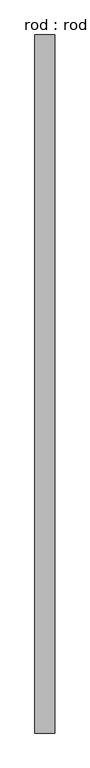
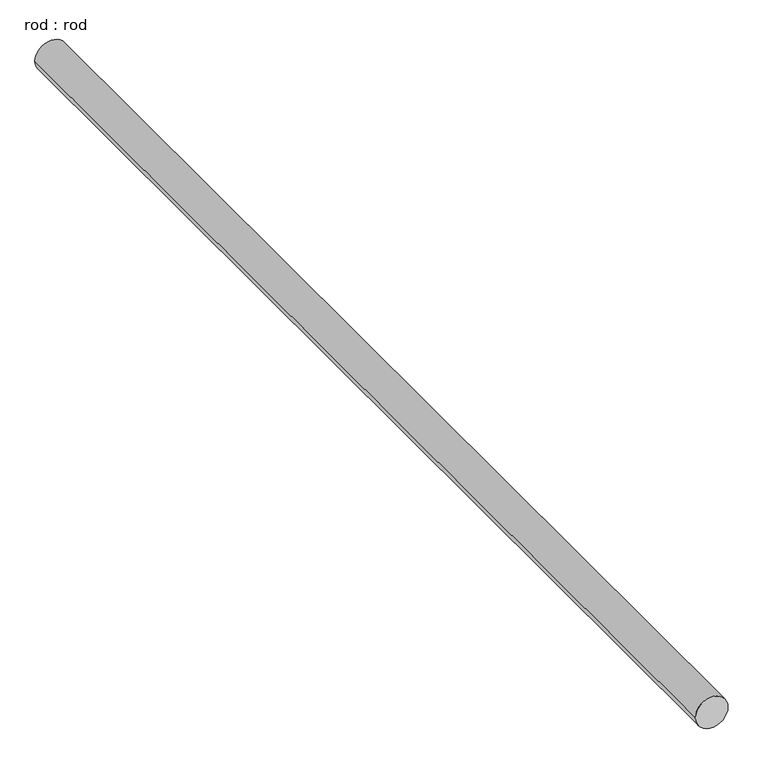
"""IFC4 building model written with IfcOpenShell, lengths in millimetres: proxy geometry, rod : rod."""

from ifc_helpers import new_model, si_unit, point, frame, frame_2d, origin, place, context, project, spatial, circle_curve, trimmed, segment, composite_curve, outline, extrude, source, transform, mapped, element, save


def rod_rod_f0030c01(model_context):
    return source(origin(), model_context, "Body", "SweptSolid", [
        extrude(outline(composite_curve([segment(trimmed(circle_curve(frame_2d((0.0108462, 0.0)), 200.0), [point((0.0108462, 200.0))], [point((0.0108462, -200.0))], False, "CARTESIAN"), True, "CONTINUOUS"), segment(trimmed(circle_curve(frame_2d((0.0108462, 0.0)), 200.0), [point((0.0108462, -200.0))], [point((0.0108462, 200.0))], False, "CARTESIAN"), True, "CONTINUOUS")], self_intersect=False)), frame((0.0, -2940.352161, 0.0), z_axis=(0.0, 1.0, 0.0), x_axis=(0.0, 0.0, 1.0)), (0.0, 0.0, 1.0), 14066.1615527),
    ])


if __name__ == "__main__":
    model = new_model("IFC4")
    model_context = context("Model", 3, world=origin())
    ifc_project = project(units=[si_unit("LENGTHUNIT", "METRE", prefix="MILLI")], contexts=[model_context])
    site = spatial("IfcSite", under=ifc_project)
    building = spatial("IfcBuilding", under=site)
    placement = place(None, origin())
    rod_rod_shape = rod_rod_f0030c01(model_context)
    element("IfcBuildingElementProxy", 1, Name="rod : rod", ObjectType="rod : rod", at=placement, inside=building, context=model_context, shape_type="MappedRepresentation", body=[
        mapped(rod_rod_shape, transform((0.0, 0.0, 0.0), x_axis=(1.0, 0.0, 0.0), y_axis=(0.0, 1.0, 0.0), z_axis=(0.0, 0.0, 1.0))),
    ])
    save(model, "model.ifc")

# Revit data of these elements
# Type "rod : rod"
#   Default Elevation = 0
